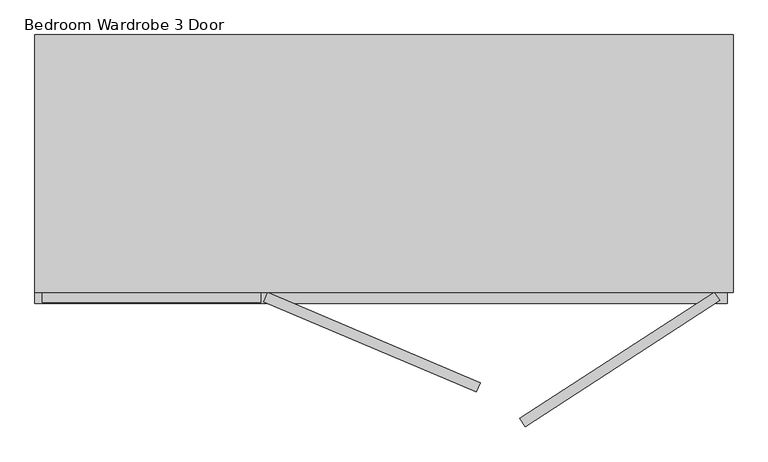
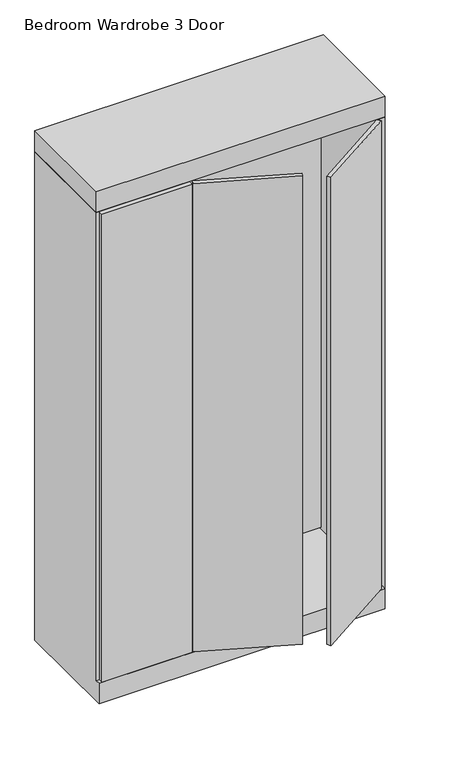
"""IFC4 building model written with IfcOpenShell, lengths in millimetres: furniture geometry, Bedroom Wardrobe 3 Door : Wardrobe 1300w x 550d x 2400h."""

import ifcopenshell
import ifcopenshell.guid

model = None  # the IFC model being written
_history = None  # IfcOwnerHistory: only IFC2X3 demands one
_inside = {}  # id of a spatial element -> (the spatial element, [elements in it])
_under = {}  # id of a project, library or spatial element -> (it, [spatial elements below it])
_declared = {}  # id of a project -> (the project, [libraries it declares])
_typed = {}  # id of a type object -> (the type object, [elements of that type])
_made_of = {}  # id of a material, layer set ... -> (it, [elements and type objects made of it])


def new_model(schema):
    """Start an empty IFC model of exactly this schema.

    Asked for "IFC4X3", IfcOpenShell would pick the latest addendum, in which some entities
    have other attributes; the version numbers below select the first issue.
    IFC2X3 requires an IfcOwnerHistory on every rooted entity: one is made here for all.
    """
    global model, _history
    if schema == "IFC4X3":
        model = ifcopenshell.file(schema_version=(4, 3, 0, 0))
    else:
        model = ifcopenshell.file(schema=schema)
    _inside.clear()
    _under.clear()
    _declared.clear()
    _typed.clear()
    _made_of.clear()
    _history = None
    if model.schema == "IFC2X3":
        org = make("IfcOrganization", Name="unknown")
        user = make(
            "IfcPersonAndOrganization",
            ThePerson=make("IfcPerson", FamilyName="unknown"),
            TheOrganization=org,
        )
        app = make(
            "IfcApplication",
            ApplicationDeveloper=org,
            Version="unknown",
            ApplicationFullName="unknown",
            ApplicationIdentifier="unknown",
        )
        _history = make(
            "IfcOwnerHistory",
            OwningUser=user,
            OwningApplication=app,
            ChangeAction="ADDED",
            CreationDate=0,
        )
    return model


def make(cls, **values):
    """One entity of the class cls with the attributes given. An attribute that is None is left unset."""
    return model.create_entity(
        cls, **{name: value for name, value in values.items() if value is not None}
    )


def rooted(cls, **values):
    """An entity with a GlobalId (a new one), such as an element, a storey or a relation."""
    return make(cls, GlobalId=ifcopenshell.guid.new(), OwnerHistory=_history, **values)


def si_unit(unit_type, name, prefix=None):
    """IfcSIUnit, for example si_unit("LENGTHUNIT", "METRE", prefix="MILLI")."""
    return make("IfcSIUnit", UnitType=unit_type, Prefix=prefix, Name=name)


def assignment(units):
    """IfcUnitAssignment: the units of a project."""
    return None if units is None else make("IfcUnitAssignment", Units=units)


def point(xyz):
    """IfcCartesianPoint."""
    return None if xyz is None else make("IfcCartesianPoint", Coordinates=xyz)


def direction(xyz):
    """IfcDirection."""
    return None if xyz is None else make("IfcDirection", DirectionRatios=xyz)


def frame(location, z_axis=None, x_axis=None):
    """IfcAxis2Placement3D, a coordinate frame: its origin and axes. An axis left out is left unset."""
    return make(
        "IfcAxis2Placement3D",
        Location=point(location),
        Axis=direction(z_axis),
        RefDirection=direction(x_axis),
    )


def origin():
    """The frame at (0, 0, 0) with its axes left unset."""
    return frame((0.0, 0.0, 0.0))


def place(relative_to, where):
    """IfcLocalPlacement: puts the frame where relative to a parent placement (None: the world)."""
    return make(
        "IfcLocalPlacement", PlacementRelTo=relative_to, RelativePlacement=where
    )


def context(
    kind, dimensions, precision=None, world=None, true_north=None, identifier=None
):
    """IfcGeometricRepresentationContext, for example the 3D "Model" context."""
    return make(
        "IfcGeometricRepresentationContext",
        ContextIdentifier=identifier,
        ContextType=kind,
        CoordinateSpaceDimension=dimensions,
        Precision=precision,
        WorldCoordinateSystem=world,
        TrueNorth=true_north,
    )


def project(units=None, contexts=None):
    """IfcProject with its units and contexts."""
    return rooted(
        "IfcProject",
        Name="project",
        RepresentationContexts=contexts,
        UnitsInContext=assignment(units),
    )


def spatial(cls, under=None, at=None, **own):
    """A site, building, storey or space (cls), placed at a placement, below another one or the project."""
    s = rooted(cls, ObjectPlacement=at, **own)
    if under is not None:
        _under.setdefault(under.id(), (under, []))[1].append(s)
    return s


def polyline(points):
    """IfcPolyline through the points."""
    return make("IfcPolyline", Points=[point(p) for p in points])


def outline(outer, holes=None, kind="AREA"):
    """IfcArbitraryClosedProfileDef: a profile drawn as a closed curve; with holes, ...WithVoids."""
    if holes is None:
        return make("IfcArbitraryClosedProfileDef", ProfileType=kind, OuterCurve=outer)
    return make(
        "IfcArbitraryProfileDefWithVoids",
        ProfileType=kind,
        OuterCurve=outer,
        InnerCurves=holes,
    )


def extrude(swept, where, along, depth):
    """IfcExtrudedAreaSolid: the profile swept, set in the frame where, extruded along a direction by depth."""
    return make(
        "IfcExtrudedAreaSolid",
        SweptArea=swept,
        Position=where,
        ExtrudedDirection=direction(along),
        Depth=depth,
    )


def faces_of(points, faces, orient=None, outer=None):
    """IfcFace entities. A face is a list of loops; a loop is a list of indices into points, from 0.

    orient and outer hold one flag for each loop. By default every Orientation is true, the
    first loop of a face is its IfcFaceOuterBound and the others are IfcFaceBound.
    """
    made = []
    for i, loops in enumerate(faces):
        bounds = []
        for j, loop in enumerate(loops):
            is_outer = j == 0 if outer is None else outer[i][j]
            bounds.append(
                make(
                    "IfcFaceOuterBound" if is_outer else "IfcFaceBound",
                    Bound=make("IfcPolyLoop", Polygon=[points[k] for k in loop]),
                    Orientation=True if orient is None else orient[i][j],
                )
            )
        made.append(make("IfcFace", Bounds=bounds))
    return made


def faceted_brep(points, faces, orient=None, outer=None, voids=None):
    """IfcFacetedBrep: a solid bounded by flat faces; with voids (closed shells), ...WithVoids."""
    shared = [point(p) for p in points]
    hull = make("IfcClosedShell", CfsFaces=faces_of(shared, faces, orient, outer))
    if voids is None:
        return make("IfcFacetedBrep", Outer=hull)
    return make(
        "IfcFacetedBrepWithVoids",
        Outer=hull,
        Voids=[
            make(cls, CfsFaces=faces_of(shared, fs, o, b)) for cls, fs, o, b in voids
        ],
    )


def shape(context_of_items, identifier, shape_type, items):
    """IfcShapeRepresentation: the items that make up one representation, for example the "Body"."""
    return make(
        "IfcShapeRepresentation",
        ContextOfItems=context_of_items,
        RepresentationIdentifier=identifier,
        RepresentationType=shape_type,
        Items=items,
    )


def source(mapping_origin, context_of_items, identifier, shape_type, items):
    """IfcRepresentationMap: a shape defined once, which mapped items show again and again."""
    return make(
        "IfcRepresentationMap",
        MappingOrigin=mapping_origin,
        MappedRepresentation=shape(context_of_items, identifier, shape_type, items),
    )


def transform(
    local_origin,
    x_axis=None,
    y_axis=None,
    z_axis=None,
    scale=None,
    scale2=None,
    scale3=None,
    uniform=True,
):
    """IfcCartesianTransformationOperator3D, or its non-uniform kind. x_axis, y_axis, z_axis: its Axis1, 2, 3."""
    if uniform:
        return make(
            "IfcCartesianTransformationOperator3D",
            Axis1=direction(x_axis),
            Axis2=direction(y_axis),
            LocalOrigin=point(local_origin),
            Scale=scale,
            Axis3=direction(z_axis),
        )
    return make(
        "IfcCartesianTransformationOperator3DnonUniform",
        Axis1=direction(x_axis),
        Axis2=direction(y_axis),
        LocalOrigin=point(local_origin),
        Scale=scale,
        Axis3=direction(z_axis),
        Scale2=scale2,
        Scale3=scale3,
    )


def mapped(mapping_source, mapping_target):
    """IfcMappedItem: shows the shape of a source again, moved by a transform."""
    return make(
        "IfcMappedItem", MappingSource=mapping_source, MappingTarget=mapping_target
    )


def made_of(thing, what):
    """Note that an element or type object is made of a material, layer set ...; save() writes the relation."""
    if what is not None:
        _made_of.setdefault(what.id(), (what, []))[1].append(thing)
    return thing


def element(
    cls,
    number,
    at=None,
    inside=None,
    cuts=None,
    type_object=None,
    material=None,
    context=None,
    identifier="Body",
    shape_type=None,
    held_by="IfcProductDefinitionShape",
    body=None,
    shapes=None,
    **own,
):
    """One element of the class cls, such as IfcWall. Its Tag is "e" and its number.

    at: its placement. inside: the storey or other place that contains it. cuts: it is an
    opening in that element (IfcRelVoidsElement). A single representation is given by context,
    identifier, shape_type and body (its items); several are given by shapes. held_by: the class
    of the entity that holds the representations. save() writes the other relations.
    """
    e = rooted(cls, Tag="e%d" % number, ObjectPlacement=at, **own)
    if body is not None:
        shapes = [shape(context, identifier, shape_type, body)]
    if shapes is not None:
        e.Representation = make(held_by, Representations=shapes)
    if inside is not None:
        _inside.setdefault(inside.id(), (inside, []))[1].append(e)
    if cuts is not None:
        rooted(
            "IfcRelVoidsElement", RelatingBuildingElement=cuts, RelatedOpeningElement=e
        )
    if type_object is not None:
        _typed.setdefault(type_object.id(), (type_object, []))[1].append(e)
    return made_of(e, material)


def aggregate(whole, parts):
    """IfcRelAggregates: a whole, such as a stair, and the parts it consists of."""
    return rooted("IfcRelAggregates", RelatingObject=whole, RelatedObjects=parts)


def save(model, path):
    """Write the relations noted so far, then the file.

    IfcRelAggregates (storeys below a building ...), IfcRelContainedInSpatialStructure (elements
    in a storey), IfcRelDefinesByType, IfcRelAssociatesMaterial and IfcRelDeclares: one each for
    every whole, place, type object, material and project.
    """
    for whole, parts in _under.values():
        aggregate(whole, parts)
    for where, things in _inside.values():
        rooted(
            "IfcRelContainedInSpatialStructure",
            RelatedElements=things,
            RelatingStructure=where,
        )
    for kind, things in _typed.values():
        rooted("IfcRelDefinesByType", RelatedObjects=things, RelatingType=kind)
    for what, things in _made_of.values():
        rooted("IfcRelAssociatesMaterial", RelatedObjects=things, RelatingMaterial=what)
    for by, libraries in _declared.values():
        rooted("IfcRelDeclares", RelatingContext=by, RelatedDefinitions=libraries)
    model.write(path)


def bedroom_wardrobe_3_door_29ed634a(model_context):
    return source(origin(), model_context, "Body", "SolidModel", [
        extrude(outline(polyline([(338.8274532, -299.1040904), (-63.5175473, -128.3187703), (-56.0741193, -110.7831528), (346.2708812, -281.568473), (338.8274532, -299.1040904)])), frame((0.0, 0.0, 111.125), z_axis=(0.0, 0.0, 1.0), x_axis=(1.0, 0.0, 0.0)), (0.0, 0.0, 1.0), 2263.775),
        extrude(outline(polyline([(798.9376868, -125.9517987), (431.030381, -364.8735967), (420.6550073, -348.8969224), (788.5623132, -109.9751244), (798.9376868, -125.9517987)])), frame((0.0, 0.0, 111.125), z_axis=(0.0, 0.0, 1.0), x_axis=(1.0, 0.0, 0.0)), (0.0, 0.0, 1.0), 2263.775),
        extrude(outline(polyline([(-69.3208333, -129.0759615), (-482.6, -129.0759615), (-482.6, -110.0259615), (-69.3208333, -110.0259615), (-69.3208333, -129.0759615)])), frame((0.0, 0.0, 111.125), z_axis=(0.0, 0.0, 1.0), x_axis=(1.0, 0.0, 0.0)), (0.0, 0.0, 1.0), 2263.775),
        faceted_brep([(-471.0843944, -110.0894509, 2374.9), (-496.4843944, -110.0894509, 2374.9), (-496.4843944, -110.0894509, 111.125), (-471.0843944, -110.0894509, 111.125), (824.3156056, -110.0894509, 26.9875), (824.3156056, -110.0894509, 2374.9), (798.9156056, -110.0894509, 2374.9), (798.9156056, -110.0894509, 111.125), (812.8, -110.0894509, 111.125), (812.8, -110.0894509, 26.9875), (824.3156056, 377.3365385, 2374.9), (824.3156056, 377.3365385, 26.9875), (812.8, 377.3365385, 26.9875), (812.8, 377.3365385, 12.7), (-496.4843944, 377.3365385, 12.7), (-496.4843944, 377.3365385, 2374.9), (-471.0843944, 377.3365385, 120.65), (-471.0843944, 377.3365385, 111.125), (798.9156056, 377.3365385, 111.125), (798.9156056, 377.3365385, 120.65), (-471.0843944, 351.9365385, 2374.9), (798.9156056, 351.9365385, 2374.9), (-496.4843944, -130.6634615, 12.7), (-496.4843944, -130.6634615, 111.125), (-471.0843944, 351.9365385, 120.65), (798.9156056, 351.9365385, 120.65), (812.8, -130.6634615, 12.7), (812.8, -130.6634615, 111.125)], [[[0, 1, 2, 3]], [[4, 5, 6, 7, 8, 9]], [[10, 11, 12, 13, 14, 15], [16, 17, 18, 19]], [[1, 0, 20, 21, 6, 5, 10, 15]], [[1, 15, 14, 22, 23, 2]], [[20, 0, 3, 17, 16, 24]], [[11, 4, 9, 12]], [[5, 4, 11, 10]], [[6, 21, 25, 19, 18, 7]], [[21, 20, 24, 25]], [[16, 19, 25, 24]], [[26, 13, 12, 9, 8, 27]], [[13, 26, 22, 14]], [[23, 27, 8, 7, 18, 17, 3, 2]], [[26, 27, 23, 22]]]),
        faceted_brep([(824.3156056, -110.0894509, 2376.4093197), (824.3156056, -110.0894509, 2476.5), (-496.4843944, -110.0894509, 2476.5), (-496.4843944, -110.0894509, 2376.4093197), (824.3156056, 377.3365385, 2376.4093197), (-496.4843944, 377.3365385, 2376.4093197), (-496.4843944, 377.3365385, 2476.5), (824.3156056, 377.3365385, 2476.5)], [[[0, 1, 2, 3]], [[4, 5, 6, 7]], [[1, 0, 4, 7]], [[2, 1, 7, 6]], [[3, 2, 6, 5]], [[0, 3, 5, 4]]]),
    ])


if __name__ == "__main__":
    model = new_model("IFC4")
    model_context = context("Model", 3, world=origin())
    ifc_project = project(units=[si_unit("LENGTHUNIT", "METRE", prefix="MILLI")], contexts=[model_context])
    site = spatial("IfcSite", under=ifc_project)
    building = spatial("IfcBuilding", under=site)
    placement = place(None, origin())
    bedroom_wardrobe_3_door_shape = bedroom_wardrobe_3_door_29ed634a(model_context)
    element("IfcFurniture", 1, ObjectType="Bedroom Wardrobe 3 Door : Wardrobe 1300w x 550d x 2400h", at=placement, inside=building, context=model_context, shape_type="MappedRepresentation", body=[
        mapped(bedroom_wardrobe_3_door_shape, transform((0.0, 0.0, 0.0), x_axis=(1.0, 0.0, 0.0), y_axis=(0.0, 1.0, 0.0), z_axis=(0.0, 0.0, 1.0))),
    ])
    save(model, "model.ifc")

# Revit data of these elements
# Type "Bedroom Wardrobe 3 Door : Wardrobe 1300w x 550d x 2400h"
#   URL = "www.coalesse.com"
#   Type Comments = "CODWS5268"
#   Model = "Live/Work - Denizen"
#   Manufacturer = "Coalesse"
#   Description = "Wardobe Storage Tower"
#   Width = 1320.8 mm
#   Skirting = 101.6 mm
#   Pelmet = 101.6 mm
#   Height = 2438.4 mm
#   Depth = 508 mm
#   Cost = 5253
#   Hidden Right Leg = yes
#   Hidden Left Leg = yes
#   Frame = Wood - Walnut, Natural
#   Encasement = Wood - Walnut, Natural
#   Door Panel = Wood - Mahogany
#   Default Elevation = 0
# Element 1 (IfcFurniture, "Bedroom Wardrobe 3 Door : Wardrobe 1300w x 550d x 2400h")
#   Materials on its faces: "Wood - Mahogany", "Wood - Walnut, Natural"
# Materials
#   "Wood - Walnut, Natural": class "Wood", colour RGB 122 82 53, transparency 0
#   "Wood - Mahogany": class "Wood", colour RGB 138 86 45, transparency 0
